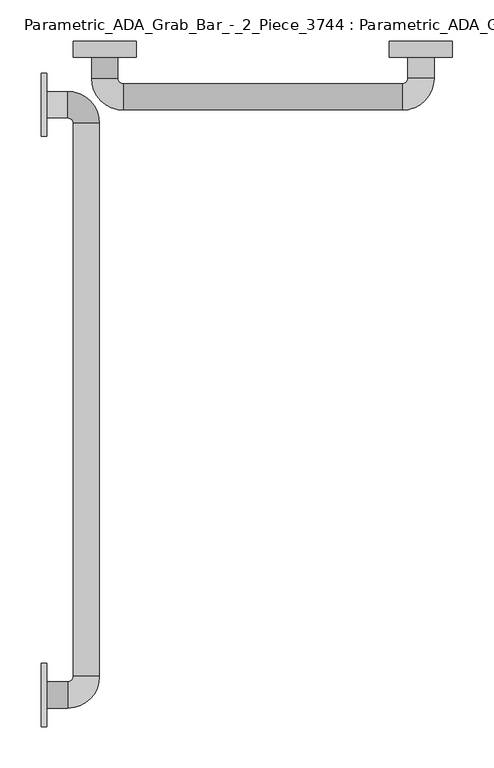
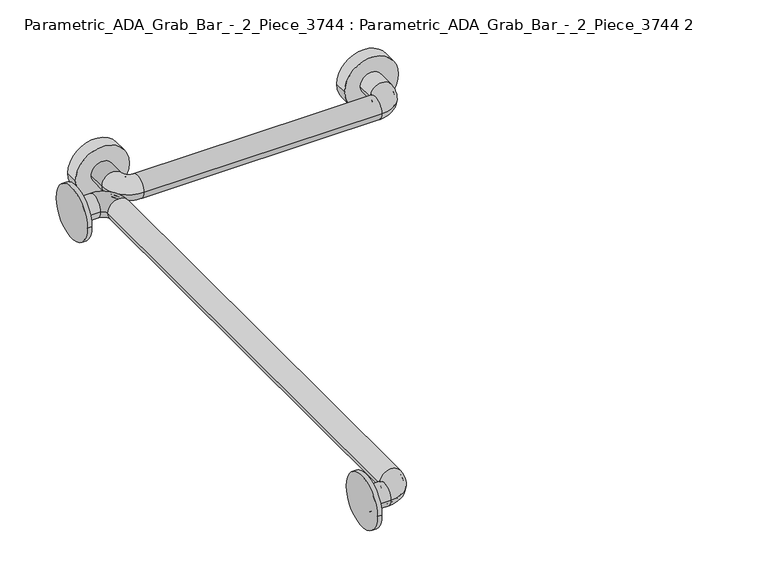
"""IFC4 building model written with IfcOpenShell, lengths in millimetres: proxy geometry, Parametric_ADA_Grab_Bar_-_2_Piece_3744 : Parametric_ADA_Grab_Bar_-_2_Piece_3744 2."""

from ifc_helpers import new_model, si_unit, point, frame, frame_2d, origin, place, context, project, spatial, polyline, circle_curve, ellipse_curve, trimmed, segment, composite_curve, outline, extrude, source, transform, mapped, element, save
from ifc_brep_helpers import plane_surface, cylinder_surface, revolved_surface, advanced_brep


def parametric_ada_grab_bar_2_piece_3744_parametric_ada_grab_bar_3060b96b(model_context):
    return source(origin(), model_context, "Body", "SolidModel", [
        advanced_brep(
        [(6.35, -828.675, 838.2), (6.35, -860.425, 838.2), (6.35, -831.85, 838.2), (6.35, -857.25, 838.2), (31.75, -860.425, 838.2), (31.75, -828.675, 838.2), (31.75, -857.25, 838.2), (31.75, -831.85, 838.2), (69.85, -822.325, 838.2), (38.1, -822.325, 838.2), (66.675, -822.325, 838.2), (41.275, -822.325, 838.2), (69.85, -155.575, 838.2), (38.1, -155.575, 838.2), (66.675, -155.575, 838.2), (41.275, -155.575, 838.2), (31.75, -117.475, 838.2), (31.75, -149.225, 838.2), (31.75, -120.65, 838.2), (31.75, -146.05, 838.2), (6.35, -149.225, 838.2), (6.35, -117.475, 838.2), (6.35, -146.05, 838.2), (6.35, -120.65, 838.2)],
        [
            (0, 1, circle_curve(frame((6.35, -844.55, 838.2), z_axis=(-1.0, 0.0, 0.0), x_axis=(0.0, -1.0, 0.0)), 15.875)),
            (1, 0, circle_curve(frame((6.35, -844.55, 838.2), z_axis=(-1.0, 0.0, 0.0), x_axis=(0.0, -1.0, 0.0)), 15.875)),
            (2, 3, circle_curve(frame((6.35, -844.55, 838.2), z_axis=(1.0, 0.0, 0.0), x_axis=(0.0, -1.0, 0.0)), 12.7)),
            (3, 2, circle_curve(frame((6.35, -844.55, 838.2), z_axis=(1.0, 0.0, 0.0), x_axis=(0.0, -1.0, 0.0)), 12.7)),
            (1, 4),
            (4, 5, circle_curve(frame((31.75, -844.55, 838.2), z_axis=(-1.0, 0.0, 0.0), x_axis=(0.0, -1.0, 0.0)), 15.875)),
            (5, 0),
            (5, 4, circle_curve(frame((31.75, -844.55, 838.2), z_axis=(-1.0, 0.0, 0.0), x_axis=(0.0, -1.0, 0.0)), 15.875)),
            (3, 6),
            (6, 7, circle_curve(frame((31.75, -844.55, 838.2), z_axis=(1.0, 0.0, 0.0), x_axis=(0.0, -1.0, 0.0)), 12.7)),
            (7, 2),
            (7, 6, circle_curve(frame((31.75, -844.55, 838.2), z_axis=(1.0, 0.0, 0.0), x_axis=(0.0, -1.0, 0.0)), 12.7)),
            (8, 9, circle_curve(frame((53.975, -822.325, 838.2), z_axis=(0.0, -1.0, 0.0), x_axis=(1.0, 0.0, 0.0)), 15.875)),
            (9, 5, circle_curve(frame((31.75, -822.325, 838.2), z_axis=(0.0, 0.0, -1.0), x_axis=(0.0, -1.0, 0.0)), 6.35)),
            (4, 8, circle_curve(frame((31.75, -822.325, 838.2), z_axis=(0.0, 0.0, 1.0), x_axis=(0.0, -1.0, 0.0)), 38.1)),
            (9, 8, circle_curve(frame((53.975, -822.325, 838.2), z_axis=(0.0, -1.0, 0.0), x_axis=(1.0, 0.0, 0.0)), 15.875)),
            (10, 11, circle_curve(frame((53.975, -822.325, 838.2), z_axis=(0.0, 1.0, 0.0), x_axis=(1.0, 0.0, 0.0)), 12.7)),
            (11, 7, circle_curve(frame((31.75, -822.325, 838.2), z_axis=(0.0, 0.0, -1.0), x_axis=(0.0, -1.0, 0.0)), 9.525)),
            (6, 10, circle_curve(frame((31.75, -822.325, 838.2), z_axis=(0.0, 0.0, 1.0), x_axis=(0.0, -1.0, 0.0)), 34.925)),
            (11, 10, circle_curve(frame((53.975, -822.325, 838.2), z_axis=(0.0, 1.0, 0.0), x_axis=(1.0, 0.0, 0.0)), 12.7)),
            (8, 12),
            (12, 13, circle_curve(frame((53.975, -155.575, 838.2), z_axis=(0.0, -1.0, 0.0), x_axis=(1.0, 0.0, 0.0)), 15.875)),
            (13, 9),
            (13, 12, circle_curve(frame((53.975, -155.575, 838.2), z_axis=(0.0, -1.0, 0.0), x_axis=(1.0, 0.0, 0.0)), 15.875)),
            (10, 14),
            (14, 15, circle_curve(frame((53.975, -155.575, 838.2), z_axis=(0.0, 1.0, 0.0), x_axis=(1.0, 0.0, 0.0)), 12.7)),
            (15, 11),
            (15, 14, circle_curve(frame((53.975, -155.575, 838.2), z_axis=(0.0, 1.0, 0.0), x_axis=(1.0, 0.0, 0.0)), 12.7)),
            (16, 17, circle_curve(frame((31.75, -133.35, 838.2), z_axis=(1.0, 0.0, 0.0), x_axis=(0.0, 1.0, 0.0)), 15.875)),
            (17, 13, circle_curve(frame((31.75, -155.575, 838.2), z_axis=(0.0, 0.0, -1.0), x_axis=(1.0, 0.0, 0.0)), 6.35)),
            (12, 16, circle_curve(frame((31.75, -155.575, 838.2), z_axis=(0.0, 0.0, 1.0), x_axis=(1.0, 0.0, 0.0)), 38.1)),
            (17, 16, circle_curve(frame((31.75, -133.35, 838.2), z_axis=(1.0, 1.076166082976765e-12, 0.0), x_axis=(-1.076166082976765e-12, 1.0, 0.0)), 15.875)),
            (18, 19, circle_curve(frame((31.75, -133.35, 838.2), z_axis=(-1.0, 0.0, 0.0), x_axis=(0.0, 1.0, 0.0)), 12.7)),
            (19, 15, circle_curve(frame((31.75, -155.575, 838.2), z_axis=(0.0, 0.0, -1.0), x_axis=(1.0, 0.0, 0.0)), 9.525)),
            (14, 18, circle_curve(frame((31.75, -155.575, 838.2), z_axis=(0.0, 0.0, 1.0), x_axis=(1.0, 0.0, 0.0)), 34.925)),
            (19, 18, circle_curve(frame((31.75, -133.35, 838.2), z_axis=(-1.0, 0.0, 0.0), x_axis=(0.0, 1.0, 0.0)), 12.7)),
            (20, 21, circle_curve(frame((6.35, -133.35, 838.2), z_axis=(-1.0, 0.0, 0.0), x_axis=(0.0, 1.0, 0.0)), 15.875)),
            (21, 20, circle_curve(frame((6.35, -133.35, 838.2), z_axis=(-1.0, 0.0, 0.0), x_axis=(0.0, 1.0, 0.0)), 15.875)),
            (22, 23, circle_curve(frame((6.35, -133.35, 838.2), z_axis=(1.0, 0.0, 0.0), x_axis=(0.0, 1.0, 0.0)), 12.7)),
            (23, 22, circle_curve(frame((6.35, -133.35, 838.2), z_axis=(1.0, 0.0, 0.0), x_axis=(0.0, 1.0, 0.0)), 12.7)),
            (16, 21),
            (20, 17),
            (18, 23),
            (22, 19),
        ],
        [
            plane_surface(frame((6.35, -844.55, 838.2), z_axis=(-1.0, 0.0, 0.0), x_axis=(0.0, 0.0, 1.0))),
            cylinder_surface(frame((6.35, -844.55, 838.2), z_axis=(-1.0, 0.0, 0.0), x_axis=(0.0, -1.0, 0.0)), 15.875),
            revolved_surface(polyline([(31.75, -857.25, 838.2), (6.35, -857.25, 838.2)]), (6.35, -844.55, 838.2), (1.0, 0.0, 0.0)),
            revolved_surface(trimmed(ellipse_curve(frame((31.75, -844.55, 838.2), z_axis=(1.0, 0.0, 0.0), x_axis=(0.0, -1.0, 0.0)), 15.875, 15.875), [point((31.75, -828.675, 838.2))], [point((31.75, -860.425, 838.2))], True, "CARTESIAN"), (31.75, -822.325, 838.2), (0.0, 0.0, -1.0)),
            revolved_surface(trimmed(ellipse_curve(frame((31.75, -844.55, 838.2), z_axis=(1.0, 0.0, 0.0), x_axis=(0.0, -1.0, 0.0)), 15.875, 15.875), [point((31.75, -860.425, 838.2))], [point((31.75, -828.675, 838.2))], True, "CARTESIAN"), (31.75, -822.325, 838.2), (0.0, 0.0, -1.0)),
            revolved_surface(trimmed(ellipse_curve(frame((31.75, -844.55, 838.2), z_axis=(-1.0, 0.0, 0.0), x_axis=(0.0, -1.0, 0.0)), 12.7, 12.7), [point((31.75, -831.85, 838.2))], [point((31.75, -857.25, 838.2))], True, "CARTESIAN"), (31.75, -822.325, 838.2), (0.0, 0.0, -1.0)),
            revolved_surface(trimmed(ellipse_curve(frame((31.75, -844.55, 838.2), z_axis=(-1.0, 0.0, 0.0), x_axis=(0.0, -1.0, 0.0)), 12.7, 12.7), [point((31.75, -857.25, 838.2))], [point((31.75, -831.85, 838.2))], True, "CARTESIAN"), (31.75, -822.325, 838.2), (0.0, 0.0, -1.0)),
            cylinder_surface(frame((53.975, -822.325, 838.2), z_axis=(0.0, -1.0, 0.0), x_axis=(1.0, 0.0, 0.0)), 15.875),
            revolved_surface(polyline([(66.675, -155.57500000000005, 838.2), (66.675, -822.325, 838.2)]), (53.975, -822.325, 838.2), (0.0, 1.0, 0.0)),
            revolved_surface(trimmed(ellipse_curve(frame((53.975, -155.575, 838.2), z_axis=(0.0, 1.0, 0.0), x_axis=(1.0, 0.0, 0.0)), 15.875, 15.875), [point((38.1, -155.575, 838.2))], [point((69.85, -155.575, 838.2))], True, "CARTESIAN"), (31.75, -155.575, 838.2), (0.0, 0.0, -1.0)),
            revolved_surface(trimmed(ellipse_curve(frame((53.975, -155.575, 838.2), z_axis=(0.0, 1.0, 0.0), x_axis=(1.0, 0.0, 0.0)), 15.875, 15.875), [point((69.85, -155.575, 838.2))], [point((38.1, -155.575, 838.2))], True, "CARTESIAN"), (31.75, -155.575, 838.2), (0.0, 0.0, -1.0)),
            revolved_surface(trimmed(ellipse_curve(frame((53.975, -155.575, 838.2), z_axis=(0.0, -1.0, 0.0), x_axis=(1.0, 0.0, 0.0)), 12.7, 12.7), [point((41.275, -155.575, 838.2))], [point((66.675, -155.575, 838.2))], True, "CARTESIAN"), (31.75, -155.575, 838.2), (0.0, 0.0, -1.0)),
            revolved_surface(trimmed(ellipse_curve(frame((53.975, -155.575, 838.2), z_axis=(0.0, -1.0, 0.0), x_axis=(1.0, 0.0, 0.0)), 12.7, 12.7), [point((66.675, -155.575, 838.2))], [point((41.275, -155.575, 838.2))], True, "CARTESIAN"), (31.75, -155.575, 838.2), (0.0, 0.0, -1.0)),
            plane_surface(frame((6.35, -133.35, 838.2), z_axis=(-1.0, 0.0, 0.0), x_axis=(0.0, 0.0, 1.0))),
            cylinder_surface(frame((31.75, -133.35, 838.2), z_axis=(1.0, 0.0, 0.0), x_axis=(0.0, 1.0, 0.0)), 15.875),
            revolved_surface(polyline([(6.350000000000001, -120.64999999999999, 838.2), (31.75, -120.64999999999999, 838.2)]), (31.75, -133.35, 838.2), (-1.0, 0.0, 0.0)),
        ],
        [
            (0, [[1, 2], [3, 4]]),
            (1, [[5, 6, 7, -2]]),
            (1, [[-7, 8, -5, -1]]),
            (2, [[9, 10, 11, -4]]),
            (2, [[-11, 12, -9, -3]]),
            (3, [[13, 14, -6, 15]]),
            (4, [[16, -15, -8, -14]]),
            (5, [[17, 18, -10, 19]]),
            (6, [[20, -19, -12, -18]]),
            (7, [[21, 22, 23, -13]]),
            (7, [[-23, 24, -21, -16]]),
            (8, [[25, 26, 27, -17]]),
            (8, [[-27, 28, -25, -20]]),
            (9, [[29, 30, -22, 31]]),
            (10, [[32, -31, -24, -30]]),
            (11, [[33, 34, -26, 35]]),
            (12, [[36, -35, -28, -34]]),
            (13, [[37, 38], [39, 40]]),
            (14, [[41, -37, 42, -29]]),
            (14, [[-42, -38, -41, -32]]),
            (15, [[43, -39, 44, -33]]),
            (15, [[-44, -40, -43, -36]]),
        ],
    ),
        advanced_brep(
        [(92.075, -76.2, 838.2), (60.325, -76.2, 838.2), (88.9, -76.2, 838.2), (63.5, -76.2, 838.2), (60.325, -101.6, 838.2), (92.075, -101.6, 838.2), (63.5, -101.6, 838.2), (88.9, -101.6, 838.2), (98.425, -139.7, 838.2), (98.425, -107.95, 838.2), (98.425, -136.525, 838.2), (98.425, -111.125, 838.2), (434.975, -139.7, 838.2), (434.975, -107.95, 838.2), (434.975, -136.525, 838.2), (434.975, -111.125, 838.2), (473.075, -101.6, 838.2), (441.325, -101.6, 838.2), (469.9, -101.6, 838.2), (444.5, -101.6, 838.2), (441.325, -76.2, 838.2), (473.075, -76.2, 838.2), (444.5, -76.2, 838.2), (469.9, -76.2, 838.2)],
        [
            (0, 1, circle_curve(frame((76.2, -76.2, 838.2), z_axis=(0.0, 1.0, 0.0), x_axis=(-1.0, 0.0, 0.0)), 15.875)),
            (1, 0, circle_curve(frame((76.2, -76.2, 838.2), z_axis=(0.0, 1.0, 0.0), x_axis=(-1.0, 0.0, 0.0)), 15.875)),
            (2, 3, circle_curve(frame((76.2, -76.2, 838.2), z_axis=(0.0, -1.0, 0.0), x_axis=(-1.0, 0.0, 0.0)), 12.7)),
            (3, 2, circle_curve(frame((76.2, -76.2, 838.2), z_axis=(0.0, -1.0, 0.0), x_axis=(-1.0, 0.0, 0.0)), 12.7)),
            (1, 4),
            (4, 5, circle_curve(frame((76.2, -101.6, 838.2), z_axis=(0.0, 1.0, 0.0), x_axis=(-1.0, 0.0, 0.0)), 15.875)),
            (5, 0),
            (5, 4, circle_curve(frame((76.2, -101.6, 838.2), z_axis=(0.0, 1.0, 0.0), x_axis=(-1.0, 0.0, 0.0)), 15.875)),
            (3, 6),
            (6, 7, circle_curve(frame((76.2, -101.6, 838.2), z_axis=(0.0, -1.0, 0.0), x_axis=(-1.0, 0.0, 0.0)), 12.7)),
            (7, 2),
            (7, 6, circle_curve(frame((76.2, -101.6, 838.2), z_axis=(0.0, -1.0, 0.0), x_axis=(-1.0, 0.0, 0.0)), 12.7)),
            (8, 9, circle_curve(frame((98.425, -123.825, 838.2), z_axis=(-1.0, 0.0, 0.0), x_axis=(0.0, -1.0, 0.0)), 15.875)),
            (9, 5, circle_curve(frame((98.425, -101.6, 838.2), z_axis=(0.0, 0.0, -1.0), x_axis=(-1.0, 0.0, 0.0)), 6.35)),
            (4, 8, circle_curve(frame((98.425, -101.6, 838.2), z_axis=(0.0, 0.0, 1.0), x_axis=(-1.0, 0.0, 0.0)), 38.1)),
            (9, 8, circle_curve(frame((98.425, -123.825, 838.2), z_axis=(-1.0, 0.0, 0.0), x_axis=(0.0, -1.0, 0.0)), 15.875)),
            (10, 11, circle_curve(frame((98.425, -123.825, 838.2), z_axis=(1.0, 0.0, 0.0), x_axis=(0.0, -1.0, 0.0)), 12.7)),
            (11, 7, circle_curve(frame((98.425, -101.6, 838.2), z_axis=(0.0, 0.0, -1.0), x_axis=(-1.0, 0.0, 0.0)), 9.525)),
            (6, 10, circle_curve(frame((98.425, -101.6, 838.2), z_axis=(0.0, 0.0, 1.0), x_axis=(-1.0, 0.0, 0.0)), 34.925)),
            (11, 10, circle_curve(frame((98.425, -123.825, 838.2), z_axis=(1.0, 0.0, 0.0), x_axis=(0.0, -1.0, 0.0)), 12.7)),
            (8, 12),
            (12, 13, circle_curve(frame((434.975, -123.825, 838.2), z_axis=(-1.0, 0.0, 0.0), x_axis=(0.0, -1.0, 0.0)), 15.875)),
            (13, 9),
            (13, 12, circle_curve(frame((434.975, -123.825, 838.2), z_axis=(-1.0, 0.0, 0.0), x_axis=(0.0, -1.0, 0.0)), 15.875)),
            (10, 14),
            (14, 15, circle_curve(frame((434.975, -123.825, 838.2), z_axis=(1.0, 0.0, 0.0), x_axis=(0.0, -1.0, 0.0)), 12.7)),
            (15, 11),
            (15, 14, circle_curve(frame((434.975, -123.825, 838.2), z_axis=(1.0, 0.0, 0.0), x_axis=(0.0, -1.0, 0.0)), 12.7)),
            (16, 17, circle_curve(frame((457.2, -101.6, 838.2), z_axis=(0.0, -1.0, 0.0), x_axis=(1.0, 0.0, 0.0)), 15.875)),
            (17, 13, circle_curve(frame((434.975, -101.6, 838.2), z_axis=(0.0, 0.0, -1.0), x_axis=(0.0, -1.0, 0.0)), 6.35)),
            (12, 16, circle_curve(frame((434.975, -101.6, 838.2), z_axis=(0.0, 0.0, 1.0), x_axis=(0.0, -1.0, 0.0)), 38.1)),
            (17, 16, circle_curve(frame((457.2, -101.6, 838.2), z_axis=(0.0, -1.0, 0.0), x_axis=(1.0, 0.0, 0.0)), 15.875)),
            (18, 19, circle_curve(frame((457.2, -101.6, 838.2), z_axis=(0.0, 1.0, 0.0), x_axis=(1.0, 0.0, 0.0)), 12.7)),
            (19, 15, circle_curve(frame((434.975, -101.6, 838.2), z_axis=(0.0, 0.0, -1.0), x_axis=(0.0, -1.0, 0.0)), 9.525)),
            (14, 18, circle_curve(frame((434.975, -101.6, 838.2), z_axis=(0.0, 0.0, 1.0), x_axis=(0.0, -1.0, 0.0)), 34.925)),
            (19, 18, circle_curve(frame((457.2, -101.6, 838.2), z_axis=(0.0, 1.0, 0.0), x_axis=(1.0, 0.0, 0.0)), 12.7)),
            (20, 21, circle_curve(frame((457.2, -76.2, 838.2), z_axis=(0.0, 1.0, 0.0), x_axis=(1.0, 0.0, 0.0)), 15.875)),
            (21, 20, circle_curve(frame((457.2, -76.2, 838.2), z_axis=(0.0, 1.0, 0.0), x_axis=(1.0, 0.0, 0.0)), 15.875)),
            (22, 23, circle_curve(frame((457.2, -76.2, 838.2), z_axis=(0.0, -1.0, 0.0), x_axis=(1.0, 0.0, 0.0)), 12.7)),
            (23, 22, circle_curve(frame((457.2, -76.2, 838.2), z_axis=(0.0, -1.0, 0.0), x_axis=(1.0, 0.0, 0.0)), 12.7)),
            (16, 21),
            (20, 17),
            (18, 23),
            (22, 19),
        ],
        [
            plane_surface(frame((76.2, -76.2, 838.2), z_axis=(0.0, 1.0, 0.0), x_axis=(0.0, 0.0, 1.0))),
            cylinder_surface(frame((76.2, -76.2, 838.2), z_axis=(0.0, 1.0, 0.0), x_axis=(-1.0, 0.0, 0.0)), 15.875),
            revolved_surface(polyline([(63.5, -101.6, 838.2), (63.5, -76.2, 838.2)]), (76.2, -76.2, 838.2), (0.0, -1.0, 0.0)),
            revolved_surface(trimmed(ellipse_curve(frame((76.2, -101.6, 838.2), z_axis=(0.0, -1.0, 0.0), x_axis=(-1.0, 0.0, 0.0)), 15.875, 15.875), [point((92.075, -101.6, 838.2))], [point((60.325, -101.6, 838.2))], True, "CARTESIAN"), (98.425, -101.6, 838.2), (0.0, 0.0, -1.0)),
            revolved_surface(trimmed(ellipse_curve(frame((76.2, -101.6, 838.2), z_axis=(0.0, -1.0, 0.0), x_axis=(-1.0, 0.0, 0.0)), 15.875, 15.875), [point((60.325, -101.6, 838.2))], [point((92.075, -101.6, 838.2))], True, "CARTESIAN"), (98.425, -101.6, 838.2), (0.0, 0.0, -1.0)),
            revolved_surface(trimmed(ellipse_curve(frame((76.2, -101.6, 838.2), z_axis=(0.0, 1.0, 0.0), x_axis=(-1.0, 0.0, 0.0)), 12.7, 12.7), [point((88.9, -101.6, 838.2))], [point((63.5, -101.6, 838.2))], True, "CARTESIAN"), (98.425, -101.6, 838.2), (0.0, 0.0, -1.0)),
            revolved_surface(trimmed(ellipse_curve(frame((76.2, -101.6, 838.2), z_axis=(0.0, 1.0, 0.0), x_axis=(-1.0, 0.0, 0.0)), 12.7, 12.7), [point((63.5, -101.6, 838.2))], [point((88.9, -101.6, 838.2))], True, "CARTESIAN"), (98.425, -101.6, 838.2), (0.0, 0.0, -1.0)),
            cylinder_surface(frame((98.425, -123.825, 838.2), z_axis=(-1.0, 0.0, 0.0), x_axis=(0.0, -1.0, 0.0)), 15.875),
            revolved_surface(polyline([(434.975, -136.525, 838.2), (98.425, -136.525, 838.2)]), (98.425, -123.825, 838.2), (1.0, 0.0, 0.0)),
            revolved_surface(trimmed(ellipse_curve(frame((434.975, -123.825, 838.2), z_axis=(1.0, 0.0, 0.0), x_axis=(0.0, -1.0, 0.0)), 15.875, 15.875), [point((434.975, -107.95, 838.2))], [point((434.975, -139.7, 838.2))], True, "CARTESIAN"), (434.975, -101.6, 838.2), (0.0, 0.0, -1.0)),
            revolved_surface(trimmed(ellipse_curve(frame((434.975, -123.825, 838.2), z_axis=(1.0, 0.0, 0.0), x_axis=(0.0, -1.0, 0.0)), 15.875, 15.875), [point((434.975, -139.7, 838.2))], [point((434.975, -107.95, 838.2))], True, "CARTESIAN"), (434.975, -101.6, 838.2), (0.0, 0.0, -1.0)),
            revolved_surface(trimmed(ellipse_curve(frame((434.975, -123.825, 838.2), z_axis=(-1.0, 0.0, 0.0), x_axis=(0.0, -1.0, 0.0)), 12.7, 12.7), [point((434.975, -111.125, 838.2))], [point((434.975, -136.525, 838.2))], True, "CARTESIAN"), (434.975, -101.6, 838.2), (0.0, 0.0, -1.0)),
            revolved_surface(trimmed(ellipse_curve(frame((434.975, -123.825, 838.2), z_axis=(-1.0, 0.0, 0.0), x_axis=(0.0, -1.0, 0.0)), 12.7, 12.7), [point((434.975, -136.525, 838.2))], [point((434.975, -111.125, 838.2))], True, "CARTESIAN"), (434.975, -101.6, 838.2), (0.0, 0.0, -1.0)),
            plane_surface(frame((457.2, -76.2, 838.2), z_axis=(0.0, 1.0, 0.0), x_axis=(0.0, 0.0, 1.0))),
            cylinder_surface(frame((457.2, -101.6, 838.2), z_axis=(0.0, -1.0, 0.0), x_axis=(1.0, 0.0, 0.0)), 15.875),
            revolved_surface(polyline([(469.9, -76.2, 838.2), (469.9, -101.6, 838.2)]), (457.2, -101.6, 838.2), (0.0, 1.0, 0.0)),
        ],
        [
            (0, [[1, 2], [3, 4]]),
            (1, [[5, 6, 7, -2]]),
            (1, [[-7, 8, -5, -1]]),
            (2, [[9, 10, 11, -4]]),
            (2, [[-11, 12, -9, -3]]),
            (3, [[13, 14, -6, 15]]),
            (4, [[16, -15, -8, -14]]),
            (5, [[17, 18, -10, 19]]),
            (6, [[20, -19, -12, -18]]),
            (7, [[21, 22, 23, -13]]),
            (7, [[-23, 24, -21, -16]]),
            (8, [[25, 26, 27, -17]]),
            (8, [[-27, 28, -25, -20]]),
            (9, [[29, 30, -22, 31]]),
            (10, [[32, -31, -24, -30]]),
            (11, [[33, 34, -26, 35]]),
            (12, [[36, -35, -28, -34]]),
            (13, [[37, 38], [39, 40]]),
            (14, [[41, -37, 42, -29]]),
            (14, [[-42, -38, -41, -32]]),
            (15, [[43, -39, 44, -33]]),
            (15, [[-44, -40, -43, -36]]),
        ],
    ),
        extrude(outline(composite_curve([segment(trimmed(circle_curve(frame_2d((-133.35, 838.2)), 38.1), [point((-95.25, 838.2))], [point((-171.45, 838.2))], False, "CARTESIAN"), True, "CONTINUOUS"), segment(trimmed(circle_curve(frame_2d((-133.35, 838.2)), 38.1), [point((-171.45, 838.2))], [point((-95.25, 838.2))], False, "CARTESIAN"), True, "CONTINUOUS")], self_intersect=False)), frame((0.0, 0.0, 0.0), z_axis=(1.0, 0.0, 0.0), x_axis=(0.0, 1.0, 0.0)), (0.0, 0.0, 1.0), 6.35),
        extrude(outline(composite_curve([segment(trimmed(circle_curve(frame_2d((-844.55, 838.2)), 38.1), [point((-806.45, 838.2))], [point((-882.65, 838.2))], False, "CARTESIAN"), True, "CONTINUOUS"), segment(trimmed(circle_curve(frame_2d((-844.55, 838.2)), 38.1), [point((-882.65, 838.2))], [point((-806.45, 838.2))], False, "CARTESIAN"), True, "CONTINUOUS")], self_intersect=False)), frame((0.0, 0.0, 0.0), z_axis=(1.0, 0.0, 0.0), x_axis=(0.0, 1.0, 0.0)), (0.0, 0.0, 1.0), 6.35),
        extrude(outline(composite_curve([segment(trimmed(circle_curve(frame_2d((838.2, 457.2)), 38.1), [point((838.2, 495.3))], [point((838.2, 419.1))], False, "CARTESIAN"), True, "CONTINUOUS"), segment(trimmed(circle_curve(frame_2d((838.2, 457.2)), 38.1), [point((838.2, 419.1))], [point((838.2, 495.3))], False, "CARTESIAN"), True, "CONTINUOUS")], self_intersect=False)), frame((0.0, -76.2, 0.0), z_axis=(0.0, 1.0, 0.0), x_axis=(0.0, 0.0, 1.0)), (0.0, 0.0, 1.0), 19.05),
        extrude(outline(composite_curve([segment(trimmed(circle_curve(frame_2d((838.2, 76.2)), 38.1), [point((838.2, 114.3))], [point((838.2, 38.1))], False, "CARTESIAN"), True, "CONTINUOUS"), segment(trimmed(circle_curve(frame_2d((838.2, 76.2)), 38.1), [point((838.2, 38.1))], [point((838.2, 114.3))], False, "CARTESIAN"), True, "CONTINUOUS")], self_intersect=False)), frame((0.0, -76.2, 0.0), z_axis=(0.0, 1.0, 0.0), x_axis=(0.0, 0.0, 1.0)), (0.0, 0.0, 1.0), 19.05),
    ])


if __name__ == "__main__":
    model = new_model("IFC4")
    model_context = context("Model", 3, world=origin())
    ifc_project = project(units=[si_unit("LENGTHUNIT", "METRE", prefix="MILLI")], contexts=[model_context])
    site = spatial("IfcSite", under=ifc_project)
    building = spatial("IfcBuilding", under=site)
    placement = place(None, origin())
    parametric_ada_grab_bar_2_piece_3744_parametric_ada_grab_bar_shape = parametric_ada_grab_bar_2_piece_3744_parametric_ada_grab_bar_3060b96b(model_context)
    element("IfcBuildingElementProxy", 1, Name="Parametric_ADA_Grab_Bar_-_2_Piece_3744 : Parametric_ADA_Grab_Bar_-_2_Piece_3744 2", ObjectType="Parametric_ADA_Grab_Bar_-_2_Piece_3744 : Parametric_ADA_Grab_Bar_-_2_Piece_3744 2", at=placement, inside=building, context=model_context, shape_type="MappedRepresentation", body=[
        mapped(parametric_ada_grab_bar_2_piece_3744_parametric_ada_grab_bar_shape, transform((0.0, 0.0, 0.0), x_axis=(1.0, 0.0, 0.0), y_axis=(0.0, 1.0, 0.0), z_axis=(0.0, 0.0, 1.0))),
    ])
    save(model, "model.ifc")

# Revit data of these elements
# Type "Parametric_ADA_Grab_Bar_-_2_Piece_3744 : Parametric_ADA_Grab_Bar_-_2_Piece_3744 2"
#   Keynote = "M10281313.01"
#   Keynote = "M10281313.01"
#   offset from wall = 0' - 0"
#   Grab bar length (42" min) = 2' - 4"
#   Grab bar height = 2' - 9"
#   Grab bar Length (36" min) = 1' - 3"
#   Face of Wall to Grab bar (6" max) = 0' - 3"
#   Face of Wall to Grab bar (12" max) = 0' - 3"
# Element 1 (IfcBuildingElementProxy, "Parametric_ADA_Grab_Bar_-_2_Piece_3744 : Parametric_ADA_Grab_Bar_-_2_Piece_3744 2")
#   Materials on its faces: "Stainless Steel"
# Materials
#   "Stainless Steel": class "Metal", colour RGB 189 187 185, transparency 0, Description = "Stainless Steel 18/8", Cost = 0
